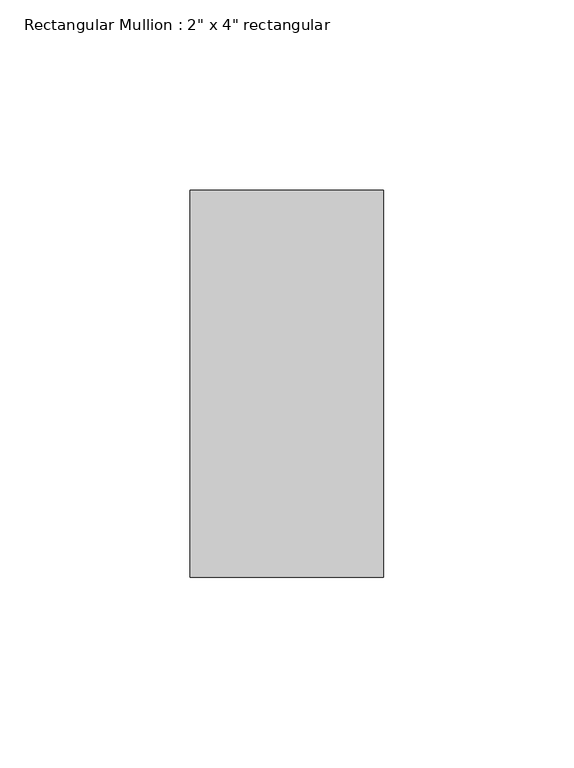
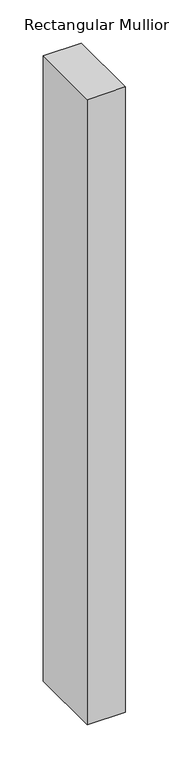
"""IFC4 building model written with IfcOpenShell, lengths in millimetres: member geometry."""

from ifc_helpers import new_model, si_unit, frame, origin, place, context, project, spatial, polyline, outline, extrude, source, transform, mapped, element, save


def member_d8235d2e(model_context):
    return source(origin(), model_context, "Body", "SweptSolid", [
        extrude(outline(polyline([(25.4, 50.8), (25.4, -50.8), (-25.4, -50.8), (-25.4, 50.8), (25.4, 50.8)])), frame((0.0, 0.0, -881.7428574), z_axis=(0.0, 0.0, 1.0), x_axis=(1.0, 0.0, 0.0)), (0.0, 0.0, 1.0), 881.7428574),
    ])


if __name__ == "__main__":
    model = new_model("IFC4")
    model_context = context("Model", 3, world=origin())
    ifc_project = project(units=[si_unit("LENGTHUNIT", "METRE", prefix="MILLI")], contexts=[model_context])
    site = spatial("IfcSite", under=ifc_project)
    building = spatial("IfcBuilding", under=site)
    placement = place(None, origin())
    member_shape = member_d8235d2e(model_context)
    element("IfcMember", 1, ObjectType="Rectangular Mullion : 2\" x 4\" rectangular", at=placement, inside=building, context=model_context, shape_type="MappedRepresentation", body=[
        mapped(member_shape, transform((0.0, 0.0, 0.0), x_axis=(1.0, 0.0, 0.0), y_axis=(0.0, 1.0, 0.0), z_axis=(0.0, 0.0, 1.0))),
    ])
    save(model, "model.ifc")

# Revit data of these elements
# Type "Rectangular Mullion : 2\" x 4\" rectangular"
#   built-in parameter 1007304 = 0.333333 (stored number, unit not read)
#   built-in parameter 1007301 = 0.0833333 (stored number, unit not read)
#   built-in parameter 1007300 = 0.0833333 (stored number, unit not read)
